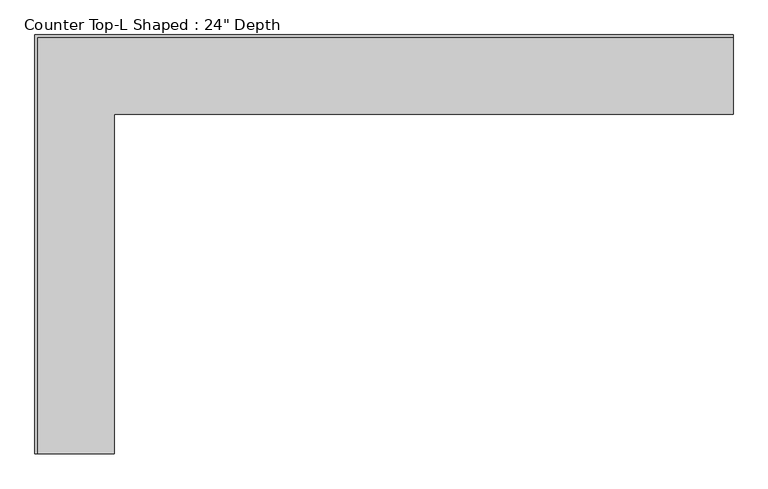
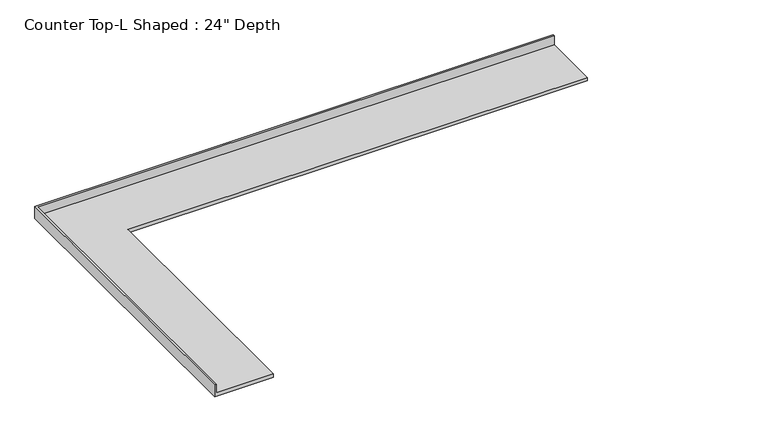
"""IFC4 building model written with IfcOpenShell, lengths in millimetres: furniture geometry."""

from ifc_helpers import new_model, si_unit, origin, place, context, project, spatial, faceted_brep, source, transform, mapped, element, save


def furniture_9bb11cb3(model_context):
    return source(origin(), model_context, "Body", "Brep", [
        faceted_brep([(-565.4622951, -3352.8, 914.4), (-565.4622951, -635.0, 914.4), (4387.5377049, -635.0, 914.4), (4387.5377049, -19.05, 914.4), (-1181.4122951, -19.05, 914.4), (-1181.4122951, -3352.8, 914.4), (4387.5377049, 0.0, 876.3), (4387.5377049, -635.0, 876.3), (-565.4622951, -635.0, 876.3), (-565.4622951, -3352.8, 876.3), (-1200.4622951, -3352.8, 876.3), (-1200.4622951, 0.0, 876.3), (-1200.4622951, 0.0, 1016.0), (4387.5377049, 0.0, 1016.0), (-1200.4622951, -3352.8, 1016.0), (-1181.4122951, -3352.8, 1016.0), (4387.5377049, -19.05, 1016.0), (-1181.4122951, -19.05, 1016.0)], [[[0, 1, 2, 3, 4, 5]], [[6, 7, 8, 9, 10, 11]], [[6, 11, 12, 13]], [[11, 10, 14, 12]], [[14, 10, 9, 0, 5, 15]], [[1, 0, 9, 8]], [[2, 1, 8, 7]], [[7, 6, 13, 16, 3, 2]], [[12, 14, 15, 17, 16, 13]], [[3, 16, 17, 4]], [[17, 15, 5, 4]]]),
    ])


if __name__ == "__main__":
    model = new_model("IFC4")
    model_context = context("Model", 3, world=origin())
    ifc_project = project(units=[si_unit("LENGTHUNIT", "METRE", prefix="MILLI")], contexts=[model_context])
    site = spatial("IfcSite", under=ifc_project)
    building = spatial("IfcBuilding", under=site)
    placement = place(None, origin())
    furniture_shape = furniture_9bb11cb3(model_context)
    element("IfcFurniture", 1, ObjectType="Counter Top-L Shaped : 24\" Depth", at=placement, inside=building, context=model_context, shape_type="MappedRepresentation", body=[
        mapped(furniture_shape, transform((0.0, 0.0, 0.0), x_axis=(1.0, 0.0, 0.0), y_axis=(0.0, 1.0, 0.0), z_axis=(0.0, 0.0, 1.0))),
    ])
    save(model, "model.ifc")

# Revit data of these elements
# Type "Counter Top-L Shaped : 24\" Depth"
#   Assembly Code = "C1030400"
#   Counter Thickness = 0' - 1 1/2"
#   Depth = 2' - 1"
#   Height = 3' - 0"
#   Length - Leg 1 [instance default] = 8' - 0"
#   Length - Leg 2 [instance default] = 6' - 0"
#   Counter Top Material = none
#   Default Elevation = 0
# Element 1 (IfcFurniture, "Counter Top-L Shaped : 24\" Depth")
#   Length - Leg 1 = 18' - 4"
#   Length - Leg 2 = 11' - 0"
#   Materials on its faces: "Counter Top"
# Materials
#   "Counter Top": class "Wood", colour RGB 226 177 128, transparency 0, Cost = 0
